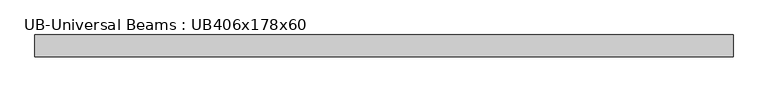
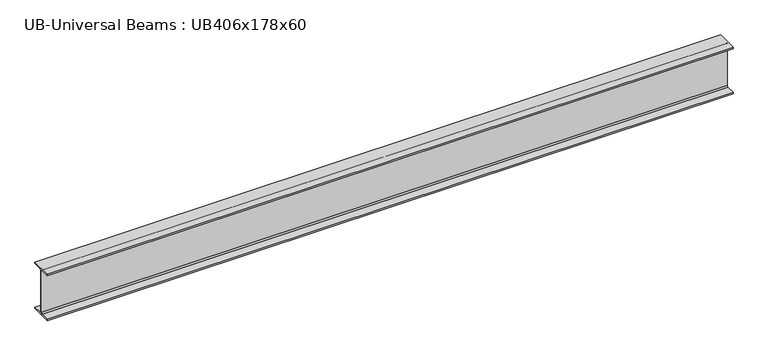
"""IFC4 building model written with IfcOpenShell, lengths in millimetres: beam geometry, UB-Universal Beams : UB406x178x60."""

from ifc_helpers import new_model, si_unit, point, frame, frame_2d, origin, place, context, project, spatial, polyline, circle_curve, trimmed, segment, composite_curve, outline, extrude, source, transform, mapped, element, save


def ub_universal_beams_ub406x178x60_ab0c7e2f(model_context):
    return source(origin(), model_context, "Body", "SweptSolid", [
        extrude(outline(composite_curve([segment(polyline([(88.95, -190.4), (88.95, -203.2), (-88.95, -203.2), (-88.95, -190.4), (-14.15, -190.4)]), True, "CONTINUOUS"), segment(trimmed(circle_curve(frame_2d((-14.15, -180.2)), 10.2), [point((-14.15, -190.4))], [point((-3.95, -180.2))], True, "CARTESIAN"), True, "CONTINUOUS"), segment(polyline([(-3.95, -180.2), (-3.95, 180.2)]), True, "CONTINUOUS"), segment(trimmed(circle_curve(frame_2d((-14.15, 180.2)), 10.2), [point((-3.95, 180.2))], [point((-14.15, 190.4))], True, "CARTESIAN"), True, "CONTINUOUS"), segment(polyline([(-14.15, 190.4), (-88.95, 190.4), (-88.95, 203.2), (88.95, 203.2), (88.95, 190.4), (14.15, 190.4)]), True, "CONTINUOUS"), segment(trimmed(circle_curve(frame_2d((14.15, 180.2)), 10.2), [point((14.15, 190.4))], [point((3.95, 180.2))], True, "CARTESIAN"), True, "CONTINUOUS"), segment(polyline([(3.95, 180.2), (3.95, -180.2)]), True, "CONTINUOUS"), segment(trimmed(circle_curve(frame_2d((14.15, -180.2)), 10.2), [point((3.95, -180.2))], [point((14.15, -190.4))], True, "CARTESIAN"), True, "CONTINUOUS"), segment(polyline([(14.15, -190.4), (88.95, -190.4)]), True, "CONTINUOUS")], self_intersect=False)), frame((-2834.6, 0.0, 0.0), z_axis=(1.0, 0.0, 0.0), x_axis=(0.0, 1.0, 0.0)), (0.0, 0.0, 1.0), 5669.2),
    ])


if __name__ == "__main__":
    model = new_model("IFC4")
    model_context = context("Model", 3, world=origin())
    ifc_project = project(units=[si_unit("LENGTHUNIT", "METRE", prefix="MILLI")], contexts=[model_context])
    site = spatial("IfcSite", under=ifc_project)
    building = spatial("IfcBuilding", under=site)
    placement = place(None, origin())
    ub_universal_beams_ub406x178x60_shape = ub_universal_beams_ub406x178x60_ab0c7e2f(model_context)
    element("IfcBeam", 1, ObjectType="UB-Universal Beams : UB406x178x60", at=placement, inside=building, context=model_context, shape_type="MappedRepresentation", body=[
        mapped(ub_universal_beams_ub406x178x60_shape, transform((0.0, 0.0, 0.0), x_axis=(1.0, 0.0, 0.0), y_axis=(0.0, 1.0, 0.0), z_axis=(0.0, 0.0, 1.0))),
    ])
    save(model, "model.ifc")

# Revit data of these elements
# Type "UB-Universal Beams : UB406x178x60"
#   Section Name Key = "UB406X178X60"
#   Width = 17.79 cm
#   Web Thickness = 0.79 cm
#   Web Fillet = 1.02 cm
#   Warping Constant = 466000.0 cm⁶
#   Torsional Moment of Inertia = 33.30 cm⁴
#   Section Area = 76.5 cm²
#   Plastic Modulus weak axis = 209.0 cm³
#   Plastic Modulus strong axis = 1200.0 cm³
#   Nominal Weight = 60.0998 kgf/m
#   Moment of Inertia weak axis = 1203.00 cm⁴
#   Moment of Inertia strong axis = 21596.00 cm⁴
#   Height = 40.64 cm
#   Flange Thickness = 1.28 cm
#   Elastic Modulus weak axis = 135.0 cm³
#   Elastic Modulus strong axis = 1063.0 cm³
#   Centroid Vertical = 20.32 cm
#   Centroid Horizontal = 8.895 cm
#   Bolt Spacing = 9.0 cm
#   Length [instance default] = 1500 mm
#   Structural Material [instance default] = Metal - Steel 43-275
#   Type Comments = ""
#   Assembly Code = ""
# Element 1 (IfcBeam, "UB-Universal Beams : UB406x178x60")
#   Materials on its faces: "Metal - Steel 43-275"
# Materials
#   "Metal - Steel 43-275": class "Metal", colour RGB 247 247 247, transparency 0, Cost = 0
